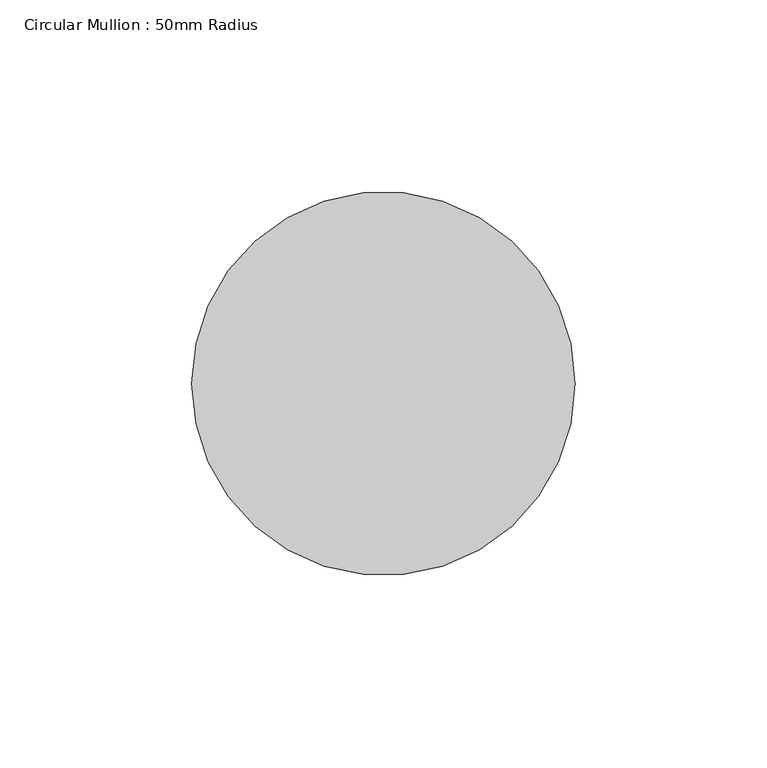
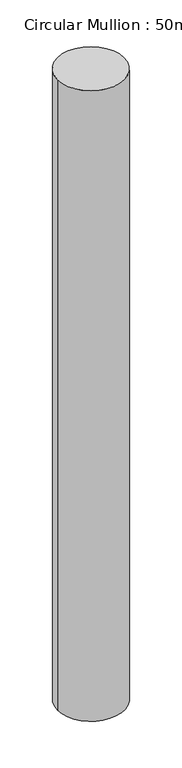
"""IFC4 building model written with IfcOpenShell, lengths in millimetres: member geometry, Circular Mullion : 50mm Radius."""

from ifc_helpers import new_model, si_unit, point, frame, origin, origin_2d, place, context, project, spatial, circle_curve, trimmed, segment, composite_curve, outline, extrude, source, transform, mapped, element, save


def circular_mullion_50mm_radius_6a36675a(model_context):
    return source(origin(), model_context, "Body", "SweptSolid", [
        extrude(outline(composite_curve([segment(trimmed(circle_curve(origin_2d(), 50.0), [point((50.0, 0.0))], [point((-50.0, 0.0))], False, "CARTESIAN"), True, "CONTINUOUS"), segment(trimmed(circle_curve(origin_2d(), 50.0), [point((-50.0, 0.0))], [point((50.0, 0.0))], False, "CARTESIAN"), True, "CONTINUOUS")], self_intersect=False)), frame((0.0, 0.0, -999.6655481), z_axis=(0.0, 0.0, 1.0), x_axis=(1.0, 0.0, 0.0)), (0.0, 0.0, 1.0), 999.6655481),
    ])


if __name__ == "__main__":
    model = new_model("IFC4")
    model_context = context("Model", 3, world=origin())
    ifc_project = project(units=[si_unit("LENGTHUNIT", "METRE", prefix="MILLI")], contexts=[model_context])
    site = spatial("IfcSite", under=ifc_project)
    building = spatial("IfcBuilding", under=site)
    placement = place(None, origin())
    circular_mullion_50mm_radius_shape = circular_mullion_50mm_radius_6a36675a(model_context)
    element("IfcMember", 1, ObjectType="Circular Mullion : 50mm Radius", at=placement, inside=building, context=model_context, shape_type="MappedRepresentation", body=[
        mapped(circular_mullion_50mm_radius_shape, transform((0.0, 0.0, 0.0), x_axis=(1.0, 0.0, 0.0), y_axis=(0.0, 1.0, 0.0), z_axis=(0.0, 0.0, 1.0))),
    ])
    save(model, "model.ifc")

# Revit data of these elements
# Type "Circular Mullion : 50mm Radius"
#   built-in parameter 1007350 = 0.164042 (stored number, unit not read)
# Element 1 (IfcMember, "Circular Mullion : 50mm Radius")
#   Materials on its faces: "Aluminium"
# Materials
#   "Aluminium": class "Metal", colour RGB 247 247 247, transparency 0, Description = "Aluminium 6061", Cost = 0
